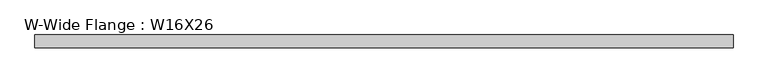
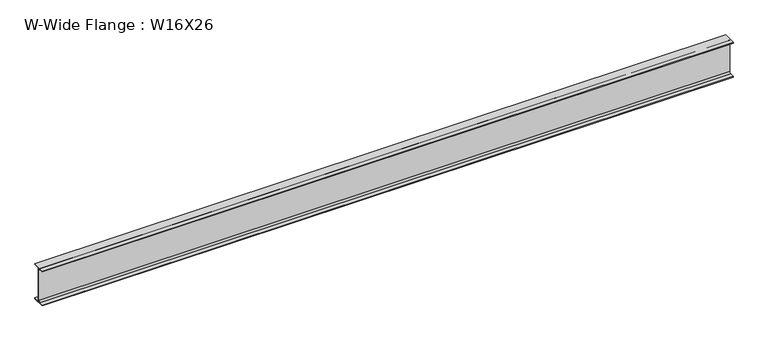
"""IFC4 building model written with IfcOpenShell, lengths in millimetres: beam geometry, W-Wide Flange : W16X26."""

from ifc_helpers import new_model, si_unit, point, frame, frame_2d, origin, place, context, project, spatial, polyline, circle_curve, trimmed, segment, composite_curve, outline, extrude, source, transform, mapped, element, save


def w_wide_flange_w16x26_a9c838cc(model_context):
    return source(origin(), model_context, "Body", "SweptSolid", [
        extrude(outline(composite_curve([segment(polyline([(69.85, -190.627), (69.85, -199.39), (-69.85, -199.39), (-69.85, -190.627), (-21.3995, -190.627)]), True, "CONTINUOUS"), segment(trimmed(circle_curve(frame_2d((-21.3995, -172.4025)), 18.2245), [point((-21.3995, -190.627))], [point((-3.175, -172.4025))], True, "CARTESIAN"), True, "CONTINUOUS"), segment(polyline([(-3.175, -172.4025), (-3.175, 172.4025)]), True, "CONTINUOUS"), segment(trimmed(circle_curve(frame_2d((-21.3995, 172.4025)), 18.2245), [point((-3.175, 172.4025))], [point((-21.3995, 190.627))], True, "CARTESIAN"), True, "CONTINUOUS"), segment(polyline([(-21.3995, 190.627), (-69.85, 190.627), (-69.85, 199.39), (69.85, 199.39), (69.85, 190.627), (21.3995, 190.627)]), True, "CONTINUOUS"), segment(trimmed(circle_curve(frame_2d((21.3995, 172.4025)), 18.2245), [point((21.3995, 190.627))], [point((3.175, 172.4025))], True, "CARTESIAN"), True, "CONTINUOUS"), segment(polyline([(3.175, 172.4025), (3.175, -172.4025)]), True, "CONTINUOUS"), segment(trimmed(circle_curve(frame_2d((21.3995, -172.4025)), 18.2245), [point((3.175, -172.4025))], [point((21.3995, -190.627))], True, "CARTESIAN"), True, "CONTINUOUS"), segment(polyline([(21.3995, -190.627), (69.85, -190.627)]), True, "CONTINUOUS")], self_intersect=False)), frame((-3654.3753906, 0.0, 0.0), z_axis=(1.0, 0.0, 0.0), x_axis=(0.0, 1.0, 0.0)), (0.0, 0.0, 1.0), 7473.1066406),
    ])


if __name__ == "__main__":
    model = new_model("IFC4")
    model_context = context("Model", 3, world=origin())
    ifc_project = project(units=[si_unit("LENGTHUNIT", "METRE", prefix="MILLI")], contexts=[model_context])
    site = spatial("IfcSite", under=ifc_project)
    building = spatial("IfcBuilding", under=site)
    placement = place(None, origin())
    w_wide_flange_w16x26_shape = w_wide_flange_w16x26_a9c838cc(model_context)
    element("IfcBeam", 1, ObjectType="W-Wide Flange : W16X26", at=placement, inside=building, context=model_context, shape_type="MappedRepresentation", body=[
        mapped(w_wide_flange_w16x26_shape, transform((0.0, 0.0, 0.0), x_axis=(1.0, 0.0, 0.0), y_axis=(0.0, 1.0, 0.0), z_axis=(0.0, 0.0, 1.0))),
    ])
    save(model, "model.ifc")

# Revit data of these elements
# Type "W-Wide Flange : W16X26"
#   Assembly Code = "B10"
#   W = 26
#   Length [instance default] = 1524 mm
#   bf = 139.7 mm
#   d = 398.78 mm
#   k = 26.988 mm
#   k2 = 18.225 mm
#   tf = 8.763 mm
#   tw = 6.35 mm
#   A = 0.00495483 m²
#   Structural Material [instance default] = Steel ASTM A992
# Element 1 (IfcBeam, "W-Wide Flange : W16X26")
#   Structural Material = Aluminum, Anodized Red
#   Materials on its faces: "Aluminum, Anodized Red"
# Materials
#   "Steel ASTM A992": class "Metal", colour RGB 128 0 0, transparency 0, Description = "Structural steel 50ksi", Cost = 0
#   "Aluminum, Anodized Red": class "Metal", colour RGB 120 120 120, transparency 0, Description = "Anodized aluminum, red", Cost = 0
